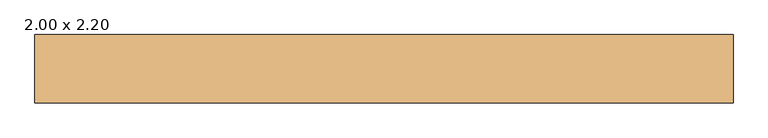
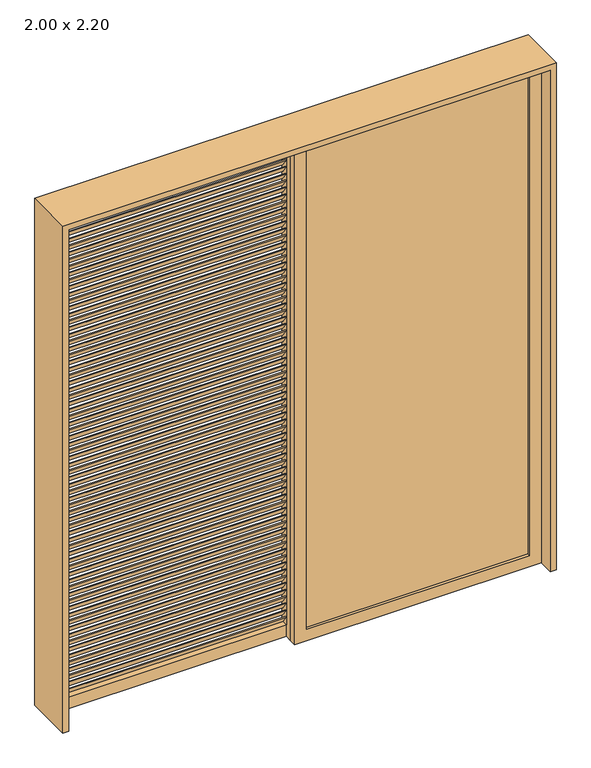
"""IFC4 building model written with IfcOpenShell, lengths in millimetres: door geometry, CC_PORTA CORRER_2 FOLHAS VENEZIANA + 1 FOLHA VIDRO : 2.00 x 2.20."""

from ifc_helpers import new_model, si_unit, frame, origin, place, context, project, spatial, polyline, outline, extrude, source, transform, mapped, element, save


def door_2_00_x_2_20_6a46caad(model_context):
    return source(origin(), model_context, "Body", "SweptSolid", [
        extrude(outline(polyline([(950.0, -26.0), (950.0, -34.0), (25.0, -34.0), (25.0, -26.0), (950.0, -26.0)])), frame((0.0, 0.0, 50.0), z_axis=(0.0, 0.0, 1.0), x_axis=(1.0, 0.0, 0.0)), (0.0, 0.0, 1.0), 2100.0),
        extrude(outline(polyline([(2200.0, 1000.0), (2200.0, -25.0), (0.0, -25.0), (0.0, 1000.0), (2200.0, 1000.0)]), holes=[polyline([(2150.0, 950.0), (50.0, 950.0), (50.0, 25.0), (2150.0, 25.0), (2150.0, 950.0)])]), frame((0.0, -45.0, 0.0), z_axis=(0.0, 1.0, 0.0), x_axis=(0.0, 0.0, 1.0)), (0.0, 0.0, 1.0), 30.0),
        extrude(outline(polyline([(40.0, 2085.0724638), (15.0, 2120.0724638), (20.0, 2120.0724638), (45.0, 2085.0724638), (40.0, 2085.0724638)])), frame((-950.0, 0.0, 0.0), z_axis=(1.0, 0.0, 0.0), x_axis=(0.0, 1.0, 0.0)), (0.0, 0.0, 1.0), 925.0),
        extrude(outline(polyline([(40.0, 2055.1449275), (15.0, 2090.1449275), (20.0, 2090.1449275), (45.0, 2055.1449275), (40.0, 2055.1449275)])), frame((-950.0, 0.0, 0.0), z_axis=(1.0, 0.0, 0.0), x_axis=(0.0, 1.0, 0.0)), (0.0, 0.0, 1.0), 925.0),
        extrude(outline(polyline([(40.0, 2025.2173913), (15.0, 2060.2173913), (20.0, 2060.2173913), (45.0, 2025.2173913), (40.0, 2025.2173913)])), frame((-950.0, 0.0, 0.0), z_axis=(1.0, 0.0, 0.0), x_axis=(0.0, 1.0, 0.0)), (0.0, 0.0, 1.0), 925.0),
        extrude(outline(polyline([(40.0, 1995.2898551), (15.0, 2030.2898551), (20.0, 2030.2898551), (45.0, 1995.2898551), (40.0, 1995.2898551)])), frame((-950.0, 0.0, 0.0), z_axis=(1.0, 0.0, 0.0), x_axis=(0.0, 1.0, 0.0)), (0.0, 0.0, 1.0), 925.0),
        extrude(outline(polyline([(40.0, 1965.3623188), (15.0, 2000.3623188), (20.0, 2000.3623188), (45.0, 1965.3623188), (40.0, 1965.3623188)])), frame((-950.0, 0.0, 0.0), z_axis=(1.0, 0.0, 0.0), x_axis=(0.0, 1.0, 0.0)), (0.0, 0.0, 1.0), 925.0),
        extrude(outline(polyline([(40.0, 1935.4347826), (15.0, 1970.4347826), (20.0, 1970.4347826), (45.0, 1935.4347826), (40.0, 1935.4347826)])), frame((-950.0, 0.0, 0.0), z_axis=(1.0, 0.0, 0.0), x_axis=(0.0, 1.0, 0.0)), (0.0, 0.0, 1.0), 925.0),
        extrude(outline(polyline([(40.0, 1905.5072464), (15.0, 1940.5072464), (20.0, 1940.5072464), (45.0, 1905.5072464), (40.0, 1905.5072464)])), frame((-950.0, 0.0, 0.0), z_axis=(1.0, 0.0, 0.0), x_axis=(0.0, 1.0, 0.0)), (0.0, 0.0, 1.0), 925.0),
        extrude(outline(polyline([(40.0, 1875.5797101), (15.0, 1910.5797101), (20.0, 1910.5797101), (45.0, 1875.5797101), (40.0, 1875.5797101)])), frame((-950.0, 0.0, 0.0), z_axis=(1.0, 0.0, 0.0), x_axis=(0.0, 1.0, 0.0)), (0.0, 0.0, 1.0), 925.0),
        extrude(outline(polyline([(40.0, 1845.6521739), (15.0, 1880.6521739), (20.0, 1880.6521739), (45.0, 1845.6521739), (40.0, 1845.6521739)])), frame((-950.0, 0.0, 0.0), z_axis=(1.0, 0.0, 0.0), x_axis=(0.0, 1.0, 0.0)), (0.0, 0.0, 1.0), 925.0),
        extrude(outline(polyline([(40.0, 1815.7246377), (15.0, 1850.7246377), (20.0, 1850.7246377), (45.0, 1815.7246377), (40.0, 1815.7246377)])), frame((-950.0, 0.0, 0.0), z_axis=(1.0, 0.0, 0.0), x_axis=(0.0, 1.0, 0.0)), (0.0, 0.0, 1.0), 925.0),
        extrude(outline(polyline([(40.0, 1785.7971014), (15.0, 1820.7971014), (20.0, 1820.7971014), (45.0, 1785.7971014), (40.0, 1785.7971014)])), frame((-950.0, 0.0, 0.0), z_axis=(1.0, 0.0, 0.0), x_axis=(0.0, 1.0, 0.0)), (0.0, 0.0, 1.0), 925.0),
        extrude(outline(polyline([(40.0, 1755.8695652), (15.0, 1790.8695652), (20.0, 1790.8695652), (45.0, 1755.8695652), (40.0, 1755.8695652)])), frame((-950.0, 0.0, 0.0), z_axis=(1.0, 0.0, 0.0), x_axis=(0.0, 1.0, 0.0)), (0.0, 0.0, 1.0), 925.0),
        extrude(outline(polyline([(40.0, 1725.942029), (15.0, 1760.942029), (20.0, 1760.942029), (45.0, 1725.942029), (40.0, 1725.942029)])), frame((-950.0, 0.0, 0.0), z_axis=(1.0, 0.0, 0.0), x_axis=(0.0, 1.0, 0.0)), (0.0, 0.0, 1.0), 925.0),
        extrude(outline(polyline([(40.0, 1696.0144928), (15.0, 1731.0144928), (20.0, 1731.0144928), (45.0, 1696.0144928), (40.0, 1696.0144928)])), frame((-950.0, 0.0, 0.0), z_axis=(1.0, 0.0, 0.0), x_axis=(0.0, 1.0, 0.0)), (0.0, 0.0, 1.0), 925.0),
        extrude(outline(polyline([(40.0, 1666.0869565), (15.0, 1701.0869565), (20.0, 1701.0869565), (45.0, 1666.0869565), (40.0, 1666.0869565)])), frame((-950.0, 0.0, 0.0), z_axis=(1.0, 0.0, 0.0), x_axis=(0.0, 1.0, 0.0)), (0.0, 0.0, 1.0), 925.0),
        extrude(outline(polyline([(40.0, 1636.1594203), (15.0, 1671.1594203), (20.0, 1671.1594203), (45.0, 1636.1594203), (40.0, 1636.1594203)])), frame((-950.0, 0.0, 0.0), z_axis=(1.0, 0.0, 0.0), x_axis=(0.0, 1.0, 0.0)), (0.0, 0.0, 1.0), 925.0),
        extrude(outline(polyline([(40.0, 1606.2318841), (15.0, 1641.2318841), (20.0, 1641.2318841), (45.0, 1606.2318841), (40.0, 1606.2318841)])), frame((-950.0, 0.0, 0.0), z_axis=(1.0, 0.0, 0.0), x_axis=(0.0, 1.0, 0.0)), (0.0, 0.0, 1.0), 925.0),
        extrude(outline(polyline([(40.0, 1576.3043478), (15.0, 1611.3043478), (20.0, 1611.3043478), (45.0, 1576.3043478), (40.0, 1576.3043478)])), frame((-950.0, 0.0, 0.0), z_axis=(1.0, 0.0, 0.0), x_axis=(0.0, 1.0, 0.0)), (0.0, 0.0, 1.0), 925.0),
        extrude(outline(polyline([(40.0, 1546.3768116), (15.0, 1581.3768116), (20.0, 1581.3768116), (45.0, 1546.3768116), (40.0, 1546.3768116)])), frame((-950.0, 0.0, 0.0), z_axis=(1.0, 0.0, 0.0), x_axis=(0.0, 1.0, 0.0)), (0.0, 0.0, 1.0), 925.0),
        extrude(outline(polyline([(40.0, 1516.4492754), (15.0, 1551.4492754), (20.0, 1551.4492754), (45.0, 1516.4492754), (40.0, 1516.4492754)])), frame((-950.0, 0.0, 0.0), z_axis=(1.0, 0.0, 0.0), x_axis=(0.0, 1.0, 0.0)), (0.0, 0.0, 1.0), 925.0),
        extrude(outline(polyline([(40.0, 1486.5217391), (15.0, 1521.5217391), (20.0, 1521.5217391), (45.0, 1486.5217391), (40.0, 1486.5217391)])), frame((-950.0, 0.0, 0.0), z_axis=(1.0, 0.0, 0.0), x_axis=(0.0, 1.0, 0.0)), (0.0, 0.0, 1.0), 925.0),
        extrude(outline(polyline([(40.0, 1456.5942029), (15.0, 1491.5942029), (20.0, 1491.5942029), (45.0, 1456.5942029), (40.0, 1456.5942029)])), frame((-950.0, 0.0, 0.0), z_axis=(1.0, 0.0, 0.0), x_axis=(0.0, 1.0, 0.0)), (0.0, 0.0, 1.0), 925.0),
        extrude(outline(polyline([(40.0, 1426.6666667), (15.0, 1461.6666667), (20.0, 1461.6666667), (45.0, 1426.6666667), (40.0, 1426.6666667)])), frame((-950.0, 0.0, 0.0), z_axis=(1.0, 0.0, 0.0), x_axis=(0.0, 1.0, 0.0)), (0.0, 0.0, 1.0), 925.0),
        extrude(outline(polyline([(40.0, 1396.7391304), (15.0, 1431.7391304), (20.0, 1431.7391304), (45.0, 1396.7391304), (40.0, 1396.7391304)])), frame((-950.0, 0.0, 0.0), z_axis=(1.0, 0.0, 0.0), x_axis=(0.0, 1.0, 0.0)), (0.0, 0.0, 1.0), 925.0),
        extrude(outline(polyline([(40.0, 1366.8115942), (15.0, 1401.8115942), (20.0, 1401.8115942), (45.0, 1366.8115942), (40.0, 1366.8115942)])), frame((-950.0, 0.0, 0.0), z_axis=(1.0, 0.0, 0.0), x_axis=(0.0, 1.0, 0.0)), (0.0, 0.0, 1.0), 925.0),
        extrude(outline(polyline([(40.0, 1336.884058), (15.0, 1371.884058), (20.0, 1371.884058), (45.0, 1336.884058), (40.0, 1336.884058)])), frame((-950.0, 0.0, 0.0), z_axis=(1.0, 0.0, 0.0), x_axis=(0.0, 1.0, 0.0)), (0.0, 0.0, 1.0), 925.0),
        extrude(outline(polyline([(40.0, 1306.9565217), (15.0, 1341.9565217), (20.0, 1341.9565217), (45.0, 1306.9565217), (40.0, 1306.9565217)])), frame((-950.0, 0.0, 0.0), z_axis=(1.0, 0.0, 0.0), x_axis=(0.0, 1.0, 0.0)), (0.0, 0.0, 1.0), 925.0),
        extrude(outline(polyline([(40.0, 1277.0289855), (15.0, 1312.0289855), (20.0, 1312.0289855), (45.0, 1277.0289855), (40.0, 1277.0289855)])), frame((-950.0, 0.0, 0.0), z_axis=(1.0, 0.0, 0.0), x_axis=(0.0, 1.0, 0.0)), (0.0, 0.0, 1.0), 925.0),
        extrude(outline(polyline([(40.0, 1247.1014493), (15.0, 1282.1014493), (20.0, 1282.1014493), (45.0, 1247.1014493), (40.0, 1247.1014493)])), frame((-950.0, 0.0, 0.0), z_axis=(1.0, 0.0, 0.0), x_axis=(0.0, 1.0, 0.0)), (0.0, 0.0, 1.0), 925.0),
        extrude(outline(polyline([(40.0, 1217.173913), (15.0, 1252.173913), (20.0, 1252.173913), (45.0, 1217.173913), (40.0, 1217.173913)])), frame((-950.0, 0.0, 0.0), z_axis=(1.0, 0.0, 0.0), x_axis=(0.0, 1.0, 0.0)), (0.0, 0.0, 1.0), 925.0),
        extrude(outline(polyline([(40.0, 1187.2463768), (15.0, 1222.2463768), (20.0, 1222.2463768), (45.0, 1187.2463768), (40.0, 1187.2463768)])), frame((-950.0, 0.0, 0.0), z_axis=(1.0, 0.0, 0.0), x_axis=(0.0, 1.0, 0.0)), (0.0, 0.0, 1.0), 925.0),
        extrude(outline(polyline([(40.0, 1157.3188406), (15.0, 1192.3188406), (20.0, 1192.3188406), (45.0, 1157.3188406), (40.0, 1157.3188406)])), frame((-950.0, 0.0, 0.0), z_axis=(1.0, 0.0, 0.0), x_axis=(0.0, 1.0, 0.0)), (0.0, 0.0, 1.0), 925.0),
        extrude(outline(polyline([(40.0, 1127.3913043), (15.0, 1162.3913043), (20.0, 1162.3913043), (45.0, 1127.3913043), (40.0, 1127.3913043)])), frame((-950.0, 0.0, 0.0), z_axis=(1.0, 0.0, 0.0), x_axis=(0.0, 1.0, 0.0)), (0.0, 0.0, 1.0), 925.0),
        extrude(outline(polyline([(40.0, 1097.4637681), (15.0, 1132.4637681), (20.0, 1132.4637681), (45.0, 1097.4637681), (40.0, 1097.4637681)])), frame((-950.0, 0.0, 0.0), z_axis=(1.0, 0.0, 0.0), x_axis=(0.0, 1.0, 0.0)), (0.0, 0.0, 1.0), 925.0),
        extrude(outline(polyline([(40.0, 1067.5362319), (15.0, 1102.5362319), (20.0, 1102.5362319), (45.0, 1067.5362319), (40.0, 1067.5362319)])), frame((-950.0, 0.0, 0.0), z_axis=(1.0, 0.0, 0.0), x_axis=(0.0, 1.0, 0.0)), (0.0, 0.0, 1.0), 925.0),
        extrude(outline(polyline([(40.0, 1037.6086957), (15.0, 1072.6086957), (20.0, 1072.6086957), (45.0, 1037.6086957), (40.0, 1037.6086957)])), frame((-950.0, 0.0, 0.0), z_axis=(1.0, 0.0, 0.0), x_axis=(0.0, 1.0, 0.0)), (0.0, 0.0, 1.0), 925.0),
        extrude(outline(polyline([(40.0, 1007.6811594), (15.0, 1042.6811594), (20.0, 1042.6811594), (45.0, 1007.6811594), (40.0, 1007.6811594)])), frame((-950.0, 0.0, 0.0), z_axis=(1.0, 0.0, 0.0), x_axis=(0.0, 1.0, 0.0)), (0.0, 0.0, 1.0), 925.0),
        extrude(outline(polyline([(40.0, 977.7536232), (15.0, 1012.7536232), (20.0, 1012.7536232), (45.0, 977.7536232), (40.0, 977.7536232)])), frame((-950.0, 0.0, 0.0), z_axis=(1.0, 0.0, 0.0), x_axis=(0.0, 1.0, 0.0)), (0.0, 0.0, 1.0), 925.0),
        extrude(outline(polyline([(40.0, 947.826087), (15.0, 982.826087), (20.0, 982.826087), (45.0, 947.826087), (40.0, 947.826087)])), frame((-950.0, 0.0, 0.0), z_axis=(1.0, 0.0, 0.0), x_axis=(0.0, 1.0, 0.0)), (0.0, 0.0, 1.0), 925.0),
        extrude(outline(polyline([(40.0, 917.8985507), (15.0, 952.8985507), (20.0, 952.8985507), (45.0, 917.8985507), (40.0, 917.8985507)])), frame((-950.0, 0.0, 0.0), z_axis=(1.0, 0.0, 0.0), x_axis=(0.0, 1.0, 0.0)), (0.0, 0.0, 1.0), 925.0),
        extrude(outline(polyline([(40.0, 887.9710145), (15.0, 922.9710145), (20.0, 922.9710145), (45.0, 887.9710145), (40.0, 887.9710145)])), frame((-950.0, 0.0, 0.0), z_axis=(1.0, 0.0, 0.0), x_axis=(0.0, 1.0, 0.0)), (0.0, 0.0, 1.0), 925.0),
        extrude(outline(polyline([(40.0, 858.0434783), (15.0, 893.0434783), (20.0, 893.0434783), (45.0, 858.0434783), (40.0, 858.0434783)])), frame((-950.0, 0.0, 0.0), z_axis=(1.0, 0.0, 0.0), x_axis=(0.0, 1.0, 0.0)), (0.0, 0.0, 1.0), 925.0),
        extrude(outline(polyline([(40.0, 828.115942), (15.0, 863.115942), (20.0, 863.115942), (45.0, 828.115942), (40.0, 828.115942)])), frame((-950.0, 0.0, 0.0), z_axis=(1.0, 0.0, 0.0), x_axis=(0.0, 1.0, 0.0)), (0.0, 0.0, 1.0), 925.0),
        extrude(outline(polyline([(40.0, 798.1884058), (15.0, 833.1884058), (20.0, 833.1884058), (45.0, 798.1884058), (40.0, 798.1884058)])), frame((-950.0, 0.0, 0.0), z_axis=(1.0, 0.0, 0.0), x_axis=(0.0, 1.0, 0.0)), (0.0, 0.0, 1.0), 925.0),
        extrude(outline(polyline([(40.0, 768.2608696), (15.0, 803.2608696), (20.0, 803.2608696), (45.0, 768.2608696), (40.0, 768.2608696)])), frame((-950.0, 0.0, 0.0), z_axis=(1.0, 0.0, 0.0), x_axis=(0.0, 1.0, 0.0)), (0.0, 0.0, 1.0), 925.0),
        extrude(outline(polyline([(40.0, 738.3333333), (15.0, 773.3333333), (20.0, 773.3333333), (45.0, 738.3333333), (40.0, 738.3333333)])), frame((-950.0, 0.0, 0.0), z_axis=(1.0, 0.0, 0.0), x_axis=(0.0, 1.0, 0.0)), (0.0, 0.0, 1.0), 925.0),
        extrude(outline(polyline([(40.0, 708.4057971), (15.0, 743.4057971), (20.0, 743.4057971), (45.0, 708.4057971), (40.0, 708.4057971)])), frame((-950.0, 0.0, 0.0), z_axis=(1.0, 0.0, 0.0), x_axis=(0.0, 1.0, 0.0)), (0.0, 0.0, 1.0), 925.0),
        extrude(outline(polyline([(40.0, 678.4782609), (15.0, 713.4782609), (20.0, 713.4782609), (45.0, 678.4782609), (40.0, 678.4782609)])), frame((-950.0, 0.0, 0.0), z_axis=(1.0, 0.0, 0.0), x_axis=(0.0, 1.0, 0.0)), (0.0, 0.0, 1.0), 925.0),
        extrude(outline(polyline([(40.0, 648.5507246), (15.0, 683.5507246), (20.0, 683.5507246), (45.0, 648.5507246), (40.0, 648.5507246)])), frame((-950.0, 0.0, 0.0), z_axis=(1.0, 0.0, 0.0), x_axis=(0.0, 1.0, 0.0)), (0.0, 0.0, 1.0), 925.0),
        extrude(outline(polyline([(40.0, 618.6231884), (15.0, 653.6231884), (20.0, 653.6231884), (45.0, 618.6231884), (40.0, 618.6231884)])), frame((-950.0, 0.0, 0.0), z_axis=(1.0, 0.0, 0.0), x_axis=(0.0, 1.0, 0.0)), (0.0, 0.0, 1.0), 925.0),
        extrude(outline(polyline([(40.0, 588.6956522), (15.0, 623.6956522), (20.0, 623.6956522), (45.0, 588.6956522), (40.0, 588.6956522)])), frame((-950.0, 0.0, 0.0), z_axis=(1.0, 0.0, 0.0), x_axis=(0.0, 1.0, 0.0)), (0.0, 0.0, 1.0), 925.0),
        extrude(outline(polyline([(40.0, 558.7681159), (15.0, 593.7681159), (20.0, 593.7681159), (45.0, 558.7681159), (40.0, 558.7681159)])), frame((-950.0, 0.0, 0.0), z_axis=(1.0, 0.0, 0.0), x_axis=(0.0, 1.0, 0.0)), (0.0, 0.0, 1.0), 925.0),
        extrude(outline(polyline([(40.0, 528.8405797), (15.0, 563.8405797), (20.0, 563.8405797), (45.0, 528.8405797), (40.0, 528.8405797)])), frame((-950.0, 0.0, 0.0), z_axis=(1.0, 0.0, 0.0), x_axis=(0.0, 1.0, 0.0)), (0.0, 0.0, 1.0), 925.0),
        extrude(outline(polyline([(40.0, 498.9130435), (15.0, 533.9130435), (20.0, 533.9130435), (45.0, 498.9130435), (40.0, 498.9130435)])), frame((-950.0, 0.0, 0.0), z_axis=(1.0, 0.0, 0.0), x_axis=(0.0, 1.0, 0.0)), (0.0, 0.0, 1.0), 925.0),
        extrude(outline(polyline([(40.0, 468.9855072), (15.0, 503.9855072), (20.0, 503.9855072), (45.0, 468.9855072), (40.0, 468.9855072)])), frame((-950.0, 0.0, 0.0), z_axis=(1.0, 0.0, 0.0), x_axis=(0.0, 1.0, 0.0)), (0.0, 0.0, 1.0), 925.0),
        extrude(outline(polyline([(40.0, 439.057971), (15.0, 474.057971), (20.0, 474.057971), (45.0, 439.057971), (40.0, 439.057971)])), frame((-950.0, 0.0, 0.0), z_axis=(1.0, 0.0, 0.0), x_axis=(0.0, 1.0, 0.0)), (0.0, 0.0, 1.0), 925.0),
        extrude(outline(polyline([(40.0, 409.1304348), (15.0, 444.1304348), (20.0, 444.1304348), (45.0, 409.1304348), (40.0, 409.1304348)])), frame((-950.0, 0.0, 0.0), z_axis=(1.0, 0.0, 0.0), x_axis=(0.0, 1.0, 0.0)), (0.0, 0.0, 1.0), 925.0),
        extrude(outline(polyline([(40.0, 379.2028986), (15.0, 414.2028986), (20.0, 414.2028986), (45.0, 379.2028986), (40.0, 379.2028986)])), frame((-950.0, 0.0, 0.0), z_axis=(1.0, 0.0, 0.0), x_axis=(0.0, 1.0, 0.0)), (0.0, 0.0, 1.0), 925.0),
        extrude(outline(polyline([(40.0, 349.2753623), (15.0, 384.2753623), (20.0, 384.2753623), (45.0, 349.2753623), (40.0, 349.2753623)])), frame((-950.0, 0.0, 0.0), z_axis=(1.0, 0.0, 0.0), x_axis=(0.0, 1.0, 0.0)), (0.0, 0.0, 1.0), 925.0),
        extrude(outline(polyline([(40.0, 319.3478261), (15.0, 354.3478261), (20.0, 354.3478261), (45.0, 319.3478261), (40.0, 319.3478261)])), frame((-950.0, 0.0, 0.0), z_axis=(1.0, 0.0, 0.0), x_axis=(0.0, 1.0, 0.0)), (0.0, 0.0, 1.0), 925.0),
        extrude(outline(polyline([(40.0, 289.4202899), (15.0, 324.4202899), (20.0, 324.4202899), (45.0, 289.4202899), (40.0, 289.4202899)])), frame((-950.0, 0.0, 0.0), z_axis=(1.0, 0.0, 0.0), x_axis=(0.0, 1.0, 0.0)), (0.0, 0.0, 1.0), 925.0),
        extrude(outline(polyline([(40.0, 259.4927536), (15.0, 294.4927536), (20.0, 294.4927536), (45.0, 259.4927536), (40.0, 259.4927536)])), frame((-950.0, 0.0, 0.0), z_axis=(1.0, 0.0, 0.0), x_axis=(0.0, 1.0, 0.0)), (0.0, 0.0, 1.0), 925.0),
        extrude(outline(polyline([(40.0, 229.5652174), (15.0, 264.5652174), (20.0, 264.5652174), (45.0, 229.5652174), (40.0, 229.5652174)])), frame((-950.0, 0.0, 0.0), z_axis=(1.0, 0.0, 0.0), x_axis=(0.0, 1.0, 0.0)), (0.0, 0.0, 1.0), 925.0),
        extrude(outline(polyline([(40.0, 199.6376812), (15.0, 234.6376812), (20.0, 234.6376812), (45.0, 199.6376812), (40.0, 199.6376812)])), frame((-950.0, 0.0, 0.0), z_axis=(1.0, 0.0, 0.0), x_axis=(0.0, 1.0, 0.0)), (0.0, 0.0, 1.0), 925.0),
        extrude(outline(polyline([(40.0, 169.7101449), (15.0, 204.7101449), (20.0, 204.7101449), (45.0, 169.7101449), (40.0, 169.7101449)])), frame((-950.0, 0.0, 0.0), z_axis=(1.0, 0.0, 0.0), x_axis=(0.0, 1.0, 0.0)), (0.0, 0.0, 1.0), 925.0),
        extrude(outline(polyline([(40.0, 139.7826087), (15.0, 174.7826087), (20.0, 174.7826087), (45.0, 139.7826087), (40.0, 139.7826087)])), frame((-950.0, 0.0, 0.0), z_axis=(1.0, 0.0, 0.0), x_axis=(0.0, 1.0, 0.0)), (0.0, 0.0, 1.0), 925.0),
        extrude(outline(polyline([(40.0, 109.8550725), (15.0, 144.8550725), (20.0, 144.8550725), (45.0, 109.8550725), (40.0, 109.8550725)])), frame((-950.0, 0.0, 0.0), z_axis=(1.0, 0.0, 0.0), x_axis=(0.0, 1.0, 0.0)), (0.0, 0.0, 1.0), 925.0),
        extrude(outline(polyline([(40.0, 79.9275362), (15.0, 114.9275362), (20.0, 114.9275362), (45.0, 79.9275362), (40.0, 79.9275362)])), frame((-950.0, 0.0, 0.0), z_axis=(1.0, 0.0, 0.0), x_axis=(0.0, 1.0, 0.0)), (0.0, 0.0, 1.0), 925.0),
        extrude(outline(polyline([(40.0, 2115.0), (15.0, 2150.0), (20.0, 2150.0), (45.0, 2115.0), (40.0, 2115.0)])), frame((-950.0, 0.0, 0.0), z_axis=(1.0, 0.0, 0.0), x_axis=(0.0, 1.0, 0.0)), (0.0, 0.0, 1.0), 925.0),
        extrude(outline(polyline([(40.0, 50.0), (15.0, 85.0), (20.0, 85.0), (45.0, 50.0), (40.0, 50.0)])), frame((-950.0, 0.0, 0.0), z_axis=(1.0, 0.0, 0.0), x_axis=(0.0, 1.0, 0.0)), (0.0, 0.0, 1.0), 925.0),
        extrude(outline(polyline([(2200.0, 25.0), (2200.0, -1000.0), (0.0, -1000.0), (0.0, 25.0), (2200.0, 25.0)]), holes=[polyline([(2150.0, -25.0), (50.0, -25.0), (50.0, -950.0), (2150.0, -950.0), (2150.0, -25.0)])]), frame((0.0, 15.0, 0.0), z_axis=(0.0, 1.0, 0.0), x_axis=(0.0, 0.0, 1.0)), (0.0, 0.0, 1.0), 30.0),
        extrude(outline(polyline([(10.0, 2085.0724638), (-15.0, 2120.0724638), (-10.0, 2120.0724638), (15.0, 2085.0724638), (10.0, 2085.0724638)])), frame((25.0, 0.0, 0.0), z_axis=(1.0, 0.0, 0.0), x_axis=(0.0, 1.0, 0.0)), (0.0, 0.0, 1.0), 925.0),
        extrude(outline(polyline([(10.0, 2055.1449275), (-15.0, 2090.1449275), (-10.0, 2090.1449275), (15.0, 2055.1449275), (10.0, 2055.1449275)])), frame((25.0, 0.0, 0.0), z_axis=(1.0, 0.0, 0.0), x_axis=(0.0, 1.0, 0.0)), (0.0, 0.0, 1.0), 925.0),
        extrude(outline(polyline([(10.0, 2025.2173913), (-15.0, 2060.2173913), (-10.0, 2060.2173913), (15.0, 2025.2173913), (10.0, 2025.2173913)])), frame((25.0, 0.0, 0.0), z_axis=(1.0, 0.0, 0.0), x_axis=(0.0, 1.0, 0.0)), (0.0, 0.0, 1.0), 925.0),
        extrude(outline(polyline([(10.0, 1995.2898551), (-15.0, 2030.2898551), (-10.0, 2030.2898551), (15.0, 1995.2898551), (10.0, 1995.2898551)])), frame((25.0, 0.0, 0.0), z_axis=(1.0, 0.0, 0.0), x_axis=(0.0, 1.0, 0.0)), (0.0, 0.0, 1.0), 925.0),
        extrude(outline(polyline([(10.0, 1965.3623188), (-15.0, 2000.3623188), (-10.0, 2000.3623188), (15.0, 1965.3623188), (10.0, 1965.3623188)])), frame((25.0, 0.0, 0.0), z_axis=(1.0, 0.0, 0.0), x_axis=(0.0, 1.0, 0.0)), (0.0, 0.0, 1.0), 925.0),
        extrude(outline(polyline([(10.0, 1935.4347826), (-15.0, 1970.4347826), (-10.0, 1970.4347826), (15.0, 1935.4347826), (10.0, 1935.4347826)])), frame((25.0, 0.0, 0.0), z_axis=(1.0, 0.0, 0.0), x_axis=(0.0, 1.0, 0.0)), (0.0, 0.0, 1.0), 925.0),
        extrude(outline(polyline([(10.0, 1905.5072464), (-15.0, 1940.5072464), (-10.0, 1940.5072464), (15.0, 1905.5072464), (10.0, 1905.5072464)])), frame((25.0, 0.0, 0.0), z_axis=(1.0, 0.0, 0.0), x_axis=(0.0, 1.0, 0.0)), (0.0, 0.0, 1.0), 925.0),
        extrude(outline(polyline([(10.0, 1875.5797101), (-15.0, 1910.5797101), (-10.0, 1910.5797101), (15.0, 1875.5797101), (10.0, 1875.5797101)])), frame((25.0, 0.0, 0.0), z_axis=(1.0, 0.0, 0.0), x_axis=(0.0, 1.0, 0.0)), (0.0, 0.0, 1.0), 925.0),
        extrude(outline(polyline([(10.0, 1845.6521739), (-15.0, 1880.6521739), (-10.0, 1880.6521739), (15.0, 1845.6521739), (10.0, 1845.6521739)])), frame((25.0, 0.0, 0.0), z_axis=(1.0, 0.0, 0.0), x_axis=(0.0, 1.0, 0.0)), (0.0, 0.0, 1.0), 925.0),
        extrude(outline(polyline([(10.0, 1815.7246377), (-15.0, 1850.7246377), (-10.0, 1850.7246377), (15.0, 1815.7246377), (10.0, 1815.7246377)])), frame((25.0, 0.0, 0.0), z_axis=(1.0, 0.0, 0.0), x_axis=(0.0, 1.0, 0.0)), (0.0, 0.0, 1.0), 925.0),
        extrude(outline(polyline([(10.0, 1785.7971014), (-15.0, 1820.7971014), (-10.0, 1820.7971014), (15.0, 1785.7971014), (10.0, 1785.7971014)])), frame((25.0, 0.0, 0.0), z_axis=(1.0, 0.0, 0.0), x_axis=(0.0, 1.0, 0.0)), (0.0, 0.0, 1.0), 925.0),
        extrude(outline(polyline([(10.0, 1755.8695652), (-15.0, 1790.8695652), (-10.0, 1790.8695652), (15.0, 1755.8695652), (10.0, 1755.8695652)])), frame((25.0, 0.0, 0.0), z_axis=(1.0, 0.0, 0.0), x_axis=(0.0, 1.0, 0.0)), (0.0, 0.0, 1.0), 925.0),
        extrude(outline(polyline([(10.0, 1725.942029), (-15.0, 1760.942029), (-10.0, 1760.942029), (15.0, 1725.942029), (10.0, 1725.942029)])), frame((25.0, 0.0, 0.0), z_axis=(1.0, 0.0, 0.0), x_axis=(0.0, 1.0, 0.0)), (0.0, 0.0, 1.0), 925.0),
        extrude(outline(polyline([(10.0, 1696.0144928), (-15.0, 1731.0144928), (-10.0, 1731.0144928), (15.0, 1696.0144928), (10.0, 1696.0144928)])), frame((25.0, 0.0, 0.0), z_axis=(1.0, 0.0, 0.0), x_axis=(0.0, 1.0, 0.0)), (0.0, 0.0, 1.0), 925.0),
        extrude(outline(polyline([(10.0, 1666.0869565), (-15.0, 1701.0869565), (-10.0, 1701.0869565), (15.0, 1666.0869565), (10.0, 1666.0869565)])), frame((25.0, 0.0, 0.0), z_axis=(1.0, 0.0, 0.0), x_axis=(0.0, 1.0, 0.0)), (0.0, 0.0, 1.0), 925.0),
        extrude(outline(polyline([(10.0, 1636.1594203), (-15.0, 1671.1594203), (-10.0, 1671.1594203), (15.0, 1636.1594203), (10.0, 1636.1594203)])), frame((25.0, 0.0, 0.0), z_axis=(1.0, 0.0, 0.0), x_axis=(0.0, 1.0, 0.0)), (0.0, 0.0, 1.0), 925.0),
        extrude(outline(polyline([(10.0, 1606.2318841), (-15.0, 1641.2318841), (-10.0, 1641.2318841), (15.0, 1606.2318841), (10.0, 1606.2318841)])), frame((25.0, 0.0, 0.0), z_axis=(1.0, 0.0, 0.0), x_axis=(0.0, 1.0, 0.0)), (0.0, 0.0, 1.0), 925.0),
        extrude(outline(polyline([(10.0, 1576.3043478), (-15.0, 1611.3043478), (-10.0, 1611.3043478), (15.0, 1576.3043478), (10.0, 1576.3043478)])), frame((25.0, 0.0, 0.0), z_axis=(1.0, 0.0, 0.0), x_axis=(0.0, 1.0, 0.0)), (0.0, 0.0, 1.0), 925.0),
        extrude(outline(polyline([(10.0, 1546.3768116), (-15.0, 1581.3768116), (-10.0, 1581.3768116), (15.0, 1546.3768116), (10.0, 1546.3768116)])), frame((25.0, 0.0, 0.0), z_axis=(1.0, 0.0, 0.0), x_axis=(0.0, 1.0, 0.0)), (0.0, 0.0, 1.0), 925.0),
        extrude(outline(polyline([(10.0, 1516.4492754), (-15.0, 1551.4492754), (-10.0, 1551.4492754), (15.0, 1516.4492754), (10.0, 1516.4492754)])), frame((25.0, 0.0, 0.0), z_axis=(1.0, 0.0, 0.0), x_axis=(0.0, 1.0, 0.0)), (0.0, 0.0, 1.0), 925.0),
        extrude(outline(polyline([(10.0, 1486.5217391), (-15.0, 1521.5217391), (-10.0, 1521.5217391), (15.0, 1486.5217391), (10.0, 1486.5217391)])), frame((25.0, 0.0, 0.0), z_axis=(1.0, 0.0, 0.0), x_axis=(0.0, 1.0, 0.0)), (0.0, 0.0, 1.0), 925.0),
        extrude(outline(polyline([(10.0, 1456.5942029), (-15.0, 1491.5942029), (-10.0, 1491.5942029), (15.0, 1456.5942029), (10.0, 1456.5942029)])), frame((25.0, 0.0, 0.0), z_axis=(1.0, 0.0, 0.0), x_axis=(0.0, 1.0, 0.0)), (0.0, 0.0, 1.0), 925.0),
        extrude(outline(polyline([(10.0, 1426.6666667), (-15.0, 1461.6666667), (-10.0, 1461.6666667), (15.0, 1426.6666667), (10.0, 1426.6666667)])), frame((25.0, 0.0, 0.0), z_axis=(1.0, 0.0, 0.0), x_axis=(0.0, 1.0, 0.0)), (0.0, 0.0, 1.0), 925.0),
        extrude(outline(polyline([(10.0, 1396.7391304), (-15.0, 1431.7391304), (-10.0, 1431.7391304), (15.0, 1396.7391304), (10.0, 1396.7391304)])), frame((25.0, 0.0, 0.0), z_axis=(1.0, 0.0, 0.0), x_axis=(0.0, 1.0, 0.0)), (0.0, 0.0, 1.0), 925.0),
        extrude(outline(polyline([(10.0, 1366.8115942), (-15.0, 1401.8115942), (-10.0, 1401.8115942), (15.0, 1366.8115942), (10.0, 1366.8115942)])), frame((25.0, 0.0, 0.0), z_axis=(1.0, 0.0, 0.0), x_axis=(0.0, 1.0, 0.0)), (0.0, 0.0, 1.0), 925.0),
        extrude(outline(polyline([(10.0, 1336.884058), (-15.0, 1371.884058), (-10.0, 1371.884058), (15.0, 1336.884058), (10.0, 1336.884058)])), frame((25.0, 0.0, 0.0), z_axis=(1.0, 0.0, 0.0), x_axis=(0.0, 1.0, 0.0)), (0.0, 0.0, 1.0), 925.0),
        extrude(outline(polyline([(10.0, 1306.9565217), (-15.0, 1341.9565217), (-10.0, 1341.9565217), (15.0, 1306.9565217), (10.0, 1306.9565217)])), frame((25.0, 0.0, 0.0), z_axis=(1.0, 0.0, 0.0), x_axis=(0.0, 1.0, 0.0)), (0.0, 0.0, 1.0), 925.0),
        extrude(outline(polyline([(10.0, 1277.0289855), (-15.0, 1312.0289855), (-10.0, 1312.0289855), (15.0, 1277.0289855), (10.0, 1277.0289855)])), frame((25.0, 0.0, 0.0), z_axis=(1.0, 0.0, 0.0), x_axis=(0.0, 1.0, 0.0)), (0.0, 0.0, 1.0), 925.0),
        extrude(outline(polyline([(10.0, 1247.1014493), (-15.0, 1282.1014493), (-10.0, 1282.1014493), (15.0, 1247.1014493), (10.0, 1247.1014493)])), frame((25.0, 0.0, 0.0), z_axis=(1.0, 0.0, 0.0), x_axis=(0.0, 1.0, 0.0)), (0.0, 0.0, 1.0), 925.0),
        extrude(outline(polyline([(10.0, 1217.173913), (-15.0, 1252.173913), (-10.0, 1252.173913), (15.0, 1217.173913), (10.0, 1217.173913)])), frame((25.0, 0.0, 0.0), z_axis=(1.0, 0.0, 0.0), x_axis=(0.0, 1.0, 0.0)), (0.0, 0.0, 1.0), 925.0),
        extrude(outline(polyline([(10.0, 1187.2463768), (-15.0, 1222.2463768), (-10.0, 1222.2463768), (15.0, 1187.2463768), (10.0, 1187.2463768)])), frame((25.0, 0.0, 0.0), z_axis=(1.0, 0.0, 0.0), x_axis=(0.0, 1.0, 0.0)), (0.0, 0.0, 1.0), 925.0),
        extrude(outline(polyline([(10.0, 1157.3188406), (-15.0, 1192.3188406), (-10.0, 1192.3188406), (15.0, 1157.3188406), (10.0, 1157.3188406)])), frame((25.0, 0.0, 0.0), z_axis=(1.0, 0.0, 0.0), x_axis=(0.0, 1.0, 0.0)), (0.0, 0.0, 1.0), 925.0),
        extrude(outline(polyline([(10.0, 1127.3913043), (-15.0, 1162.3913043), (-10.0, 1162.3913043), (15.0, 1127.3913043), (10.0, 1127.3913043)])), frame((25.0, 0.0, 0.0), z_axis=(1.0, 0.0, 0.0), x_axis=(0.0, 1.0, 0.0)), (0.0, 0.0, 1.0), 925.0),
        extrude(outline(polyline([(10.0, 1097.4637681), (-15.0, 1132.4637681), (-10.0, 1132.4637681), (15.0, 1097.4637681), (10.0, 1097.4637681)])), frame((25.0, 0.0, 0.0), z_axis=(1.0, 0.0, 0.0), x_axis=(0.0, 1.0, 0.0)), (0.0, 0.0, 1.0), 925.0),
        extrude(outline(polyline([(10.0, 1067.5362319), (-15.0, 1102.5362319), (-10.0, 1102.5362319), (15.0, 1067.5362319), (10.0, 1067.5362319)])), frame((25.0, 0.0, 0.0), z_axis=(1.0, 0.0, 0.0), x_axis=(0.0, 1.0, 0.0)), (0.0, 0.0, 1.0), 925.0),
        extrude(outline(polyline([(10.0, 1037.6086957), (-15.0, 1072.6086957), (-10.0, 1072.6086957), (15.0, 1037.6086957), (10.0, 1037.6086957)])), frame((25.0, 0.0, 0.0), z_axis=(1.0, 0.0, 0.0), x_axis=(0.0, 1.0, 0.0)), (0.0, 0.0, 1.0), 925.0),
        extrude(outline(polyline([(10.0, 1007.6811594), (-15.0, 1042.6811594), (-10.0, 1042.6811594), (15.0, 1007.6811594), (10.0, 1007.6811594)])), frame((25.0, 0.0, 0.0), z_axis=(1.0, 0.0, 0.0), x_axis=(0.0, 1.0, 0.0)), (0.0, 0.0, 1.0), 925.0),
        extrude(outline(polyline([(10.0, 977.7536232), (-15.0, 1012.7536232), (-10.0, 1012.7536232), (15.0, 977.7536232), (10.0, 977.7536232)])), frame((25.0, 0.0, 0.0), z_axis=(1.0, 0.0, 0.0), x_axis=(0.0, 1.0, 0.0)), (0.0, 0.0, 1.0), 925.0),
        extrude(outline(polyline([(10.0, 947.826087), (-15.0, 982.826087), (-10.0, 982.826087), (15.0, 947.826087), (10.0, 947.826087)])), frame((25.0, 0.0, 0.0), z_axis=(1.0, 0.0, 0.0), x_axis=(0.0, 1.0, 0.0)), (0.0, 0.0, 1.0), 925.0),
        extrude(outline(polyline([(10.0, 917.8985507), (-15.0, 952.8985507), (-10.0, 952.8985507), (15.0, 917.8985507), (10.0, 917.8985507)])), frame((25.0, 0.0, 0.0), z_axis=(1.0, 0.0, 0.0), x_axis=(0.0, 1.0, 0.0)), (0.0, 0.0, 1.0), 925.0),
        extrude(outline(polyline([(10.0, 887.9710145), (-15.0, 922.9710145), (-10.0, 922.9710145), (15.0, 887.9710145), (10.0, 887.9710145)])), frame((25.0, 0.0, 0.0), z_axis=(1.0, 0.0, 0.0), x_axis=(0.0, 1.0, 0.0)), (0.0, 0.0, 1.0), 925.0),
        extrude(outline(polyline([(10.0, 858.0434783), (-15.0, 893.0434783), (-10.0, 893.0434783), (15.0, 858.0434783), (10.0, 858.0434783)])), frame((25.0, 0.0, 0.0), z_axis=(1.0, 0.0, 0.0), x_axis=(0.0, 1.0, 0.0)), (0.0, 0.0, 1.0), 925.0),
        extrude(outline(polyline([(10.0, 828.115942), (-15.0, 863.115942), (-10.0, 863.115942), (15.0, 828.115942), (10.0, 828.115942)])), frame((25.0, 0.0, 0.0), z_axis=(1.0, 0.0, 0.0), x_axis=(0.0, 1.0, 0.0)), (0.0, 0.0, 1.0), 925.0),
        extrude(outline(polyline([(10.0, 798.1884058), (-15.0, 833.1884058), (-10.0, 833.1884058), (15.0, 798.1884058), (10.0, 798.1884058)])), frame((25.0, 0.0, 0.0), z_axis=(1.0, 0.0, 0.0), x_axis=(0.0, 1.0, 0.0)), (0.0, 0.0, 1.0), 925.0),
        extrude(outline(polyline([(10.0, 768.2608696), (-15.0, 803.2608696), (-10.0, 803.2608696), (15.0, 768.2608696), (10.0, 768.2608696)])), frame((25.0, 0.0, 0.0), z_axis=(1.0, 0.0, 0.0), x_axis=(0.0, 1.0, 0.0)), (0.0, 0.0, 1.0), 925.0),
        extrude(outline(polyline([(10.0, 738.3333333), (-15.0, 773.3333333), (-10.0, 773.3333333), (15.0, 738.3333333), (10.0, 738.3333333)])), frame((25.0, 0.0, 0.0), z_axis=(1.0, 0.0, 0.0), x_axis=(0.0, 1.0, 0.0)), (0.0, 0.0, 1.0), 925.0),
        extrude(outline(polyline([(10.0, 708.4057971), (-15.0, 743.4057971), (-10.0, 743.4057971), (15.0, 708.4057971), (10.0, 708.4057971)])), frame((25.0, 0.0, 0.0), z_axis=(1.0, 0.0, 0.0), x_axis=(0.0, 1.0, 0.0)), (0.0, 0.0, 1.0), 925.0),
        extrude(outline(polyline([(10.0, 678.4782609), (-15.0, 713.4782609), (-10.0, 713.4782609), (15.0, 678.4782609), (10.0, 678.4782609)])), frame((25.0, 0.0, 0.0), z_axis=(1.0, 0.0, 0.0), x_axis=(0.0, 1.0, 0.0)), (0.0, 0.0, 1.0), 925.0),
        extrude(outline(polyline([(10.0, 648.5507246), (-15.0, 683.5507246), (-10.0, 683.5507246), (15.0, 648.5507246), (10.0, 648.5507246)])), frame((25.0, 0.0, 0.0), z_axis=(1.0, 0.0, 0.0), x_axis=(0.0, 1.0, 0.0)), (0.0, 0.0, 1.0), 925.0),
        extrude(outline(polyline([(10.0, 618.6231884), (-15.0, 653.6231884), (-10.0, 653.6231884), (15.0, 618.6231884), (10.0, 618.6231884)])), frame((25.0, 0.0, 0.0), z_axis=(1.0, 0.0, 0.0), x_axis=(0.0, 1.0, 0.0)), (0.0, 0.0, 1.0), 925.0),
        extrude(outline(polyline([(10.0, 588.6956522), (-15.0, 623.6956522), (-10.0, 623.6956522), (15.0, 588.6956522), (10.0, 588.6956522)])), frame((25.0, 0.0, 0.0), z_axis=(1.0, 0.0, 0.0), x_axis=(0.0, 1.0, 0.0)), (0.0, 0.0, 1.0), 925.0),
        extrude(outline(polyline([(10.0, 558.7681159), (-15.0, 593.7681159), (-10.0, 593.7681159), (15.0, 558.7681159), (10.0, 558.7681159)])), frame((25.0, 0.0, 0.0), z_axis=(1.0, 0.0, 0.0), x_axis=(0.0, 1.0, 0.0)), (0.0, 0.0, 1.0), 925.0),
        extrude(outline(polyline([(10.0, 528.8405797), (-15.0, 563.8405797), (-10.0, 563.8405797), (15.0, 528.8405797), (10.0, 528.8405797)])), frame((25.0, 0.0, 0.0), z_axis=(1.0, 0.0, 0.0), x_axis=(0.0, 1.0, 0.0)), (0.0, 0.0, 1.0), 925.0),
        extrude(outline(polyline([(10.0, 498.9130435), (-15.0, 533.9130435), (-10.0, 533.9130435), (15.0, 498.9130435), (10.0, 498.9130435)])), frame((25.0, 0.0, 0.0), z_axis=(1.0, 0.0, 0.0), x_axis=(0.0, 1.0, 0.0)), (0.0, 0.0, 1.0), 925.0),
        extrude(outline(polyline([(10.0, 468.9855072), (-15.0, 503.9855072), (-10.0, 503.9855072), (15.0, 468.9855072), (10.0, 468.9855072)])), frame((25.0, 0.0, 0.0), z_axis=(1.0, 0.0, 0.0), x_axis=(0.0, 1.0, 0.0)), (0.0, 0.0, 1.0), 925.0),
        extrude(outline(polyline([(10.0, 439.057971), (-15.0, 474.057971), (-10.0, 474.057971), (15.0, 439.057971), (10.0, 439.057971)])), frame((25.0, 0.0, 0.0), z_axis=(1.0, 0.0, 0.0), x_axis=(0.0, 1.0, 0.0)), (0.0, 0.0, 1.0), 925.0),
        extrude(outline(polyline([(10.0, 409.1304348), (-15.0, 444.1304348), (-10.0, 444.1304348), (15.0, 409.1304348), (10.0, 409.1304348)])), frame((25.0, 0.0, 0.0), z_axis=(1.0, 0.0, 0.0), x_axis=(0.0, 1.0, 0.0)), (0.0, 0.0, 1.0), 925.0),
        extrude(outline(polyline([(10.0, 379.2028986), (-15.0, 414.2028986), (-10.0, 414.2028986), (15.0, 379.2028986), (10.0, 379.2028986)])), frame((25.0, 0.0, 0.0), z_axis=(1.0, 0.0, 0.0), x_axis=(0.0, 1.0, 0.0)), (0.0, 0.0, 1.0), 925.0),
        extrude(outline(polyline([(10.0, 349.2753623), (-15.0, 384.2753623), (-10.0, 384.2753623), (15.0, 349.2753623), (10.0, 349.2753623)])), frame((25.0, 0.0, 0.0), z_axis=(1.0, 0.0, 0.0), x_axis=(0.0, 1.0, 0.0)), (0.0, 0.0, 1.0), 925.0),
        extrude(outline(polyline([(10.0, 319.3478261), (-15.0, 354.3478261), (-10.0, 354.3478261), (15.0, 319.3478261), (10.0, 319.3478261)])), frame((25.0, 0.0, 0.0), z_axis=(1.0, 0.0, 0.0), x_axis=(0.0, 1.0, 0.0)), (0.0, 0.0, 1.0), 925.0),
        extrude(outline(polyline([(10.0, 289.4202899), (-15.0, 324.4202899), (-10.0, 324.4202899), (15.0, 289.4202899), (10.0, 289.4202899)])), frame((25.0, 0.0, 0.0), z_axis=(1.0, 0.0, 0.0), x_axis=(0.0, 1.0, 0.0)), (0.0, 0.0, 1.0), 925.0),
        extrude(outline(polyline([(10.0, 259.4927536), (-15.0, 294.4927536), (-10.0, 294.4927536), (15.0, 259.4927536), (10.0, 259.4927536)])), frame((25.0, 0.0, 0.0), z_axis=(1.0, 0.0, 0.0), x_axis=(0.0, 1.0, 0.0)), (0.0, 0.0, 1.0), 925.0),
        extrude(outline(polyline([(10.0, 229.5652174), (-15.0, 264.5652174), (-10.0, 264.5652174), (15.0, 229.5652174), (10.0, 229.5652174)])), frame((25.0, 0.0, 0.0), z_axis=(1.0, 0.0, 0.0), x_axis=(0.0, 1.0, 0.0)), (0.0, 0.0, 1.0), 925.0),
        extrude(outline(polyline([(10.0, 199.6376812), (-15.0, 234.6376812), (-10.0, 234.6376812), (15.0, 199.6376812), (10.0, 199.6376812)])), frame((25.0, 0.0, 0.0), z_axis=(1.0, 0.0, 0.0), x_axis=(0.0, 1.0, 0.0)), (0.0, 0.0, 1.0), 925.0),
        extrude(outline(polyline([(10.0, 169.7101449), (-15.0, 204.7101449), (-10.0, 204.7101449), (15.0, 169.7101449), (10.0, 169.7101449)])), frame((25.0, 0.0, 0.0), z_axis=(1.0, 0.0, 0.0), x_axis=(0.0, 1.0, 0.0)), (0.0, 0.0, 1.0), 925.0),
        extrude(outline(polyline([(10.0, 139.7826087), (-15.0, 174.7826087), (-10.0, 174.7826087), (15.0, 139.7826087), (10.0, 139.7826087)])), frame((25.0, 0.0, 0.0), z_axis=(1.0, 0.0, 0.0), x_axis=(0.0, 1.0, 0.0)), (0.0, 0.0, 1.0), 925.0),
        extrude(outline(polyline([(10.0, 109.8550725), (-15.0, 144.8550725), (-10.0, 144.8550725), (15.0, 109.8550725), (10.0, 109.8550725)])), frame((25.0, 0.0, 0.0), z_axis=(1.0, 0.0, 0.0), x_axis=(0.0, 1.0, 0.0)), (0.0, 0.0, 1.0), 925.0),
        extrude(outline(polyline([(10.0, 79.9275362), (-15.0, 114.9275362), (-10.0, 114.9275362), (15.0, 79.9275362), (10.0, 79.9275362)])), frame((25.0, 0.0, 0.0), z_axis=(1.0, 0.0, 0.0), x_axis=(0.0, 1.0, 0.0)), (0.0, 0.0, 1.0), 925.0),
        extrude(outline(polyline([(10.0, 2115.0), (-15.0, 2150.0), (-10.0, 2150.0), (15.0, 2115.0), (10.0, 2115.0)])), frame((25.0, 0.0, 0.0), z_axis=(1.0, 0.0, 0.0), x_axis=(0.0, 1.0, 0.0)), (0.0, 0.0, 1.0), 925.0),
        extrude(outline(polyline([(10.0, 50.0), (-15.0, 85.0), (-10.0, 85.0), (15.0, 50.0), (10.0, 50.0)])), frame((25.0, 0.0, 0.0), z_axis=(1.0, 0.0, 0.0), x_axis=(0.0, 1.0, 0.0)), (0.0, 0.0, 1.0), 925.0),
        extrude(outline(polyline([(2200.0, 1000.0), (2200.0, -25.0), (0.0, -25.0), (0.0, 1000.0), (2200.0, 1000.0)]), holes=[polyline([(2150.0, 950.0), (50.0, 950.0), (50.0, 25.0), (2150.0, 25.0), (2150.0, 950.0)])]), frame((0.0, -15.0, 0.0), z_axis=(0.0, 1.0, 0.0), x_axis=(0.0, 0.0, 1.0)), (0.0, 0.0, 1.0), 30.0),
        extrude(outline(polyline([(0.0, -1025.0), (0.0, -1000.0), (2200.0, -1000.0), (2200.0, 1000.0), (0.0, 1000.0), (0.0, 1025.0), (2225.0, 1025.0), (2225.0, -1025.0), (0.0, -1025.0)])), frame((0.0, -107.5, 0.0), z_axis=(0.0, 1.0, 0.0), x_axis=(0.0, 0.0, 1.0)), (0.0, 0.0, 1.0), 200.0),
    ])


if __name__ == "__main__":
    model = new_model("IFC4")
    model_context = context("Model", 3, world=origin())
    ifc_project = project(units=[si_unit("LENGTHUNIT", "METRE", prefix="MILLI")], contexts=[model_context])
    site = spatial("IfcSite", under=ifc_project)
    building = spatial("IfcBuilding", under=site)
    placement = place(None, origin())
    door_2_00_x_2_20_shape = door_2_00_x_2_20_6a46caad(model_context)
    element("IfcDoor", 1, ObjectType="CC_PORTA CORRER_2 FOLHAS VENEZIANA + 1 FOLHA VIDRO : 2.00 x 2.20", at=placement, inside=building, context=model_context, shape_type="MappedRepresentation", body=[
        mapped(door_2_00_x_2_20_shape, transform((0.0, 0.0, 0.0), x_axis=(1.0, 0.0, 0.0), y_axis=(0.0, 1.0, 0.0), z_axis=(0.0, 0.0, 1.0))),
    ])
    save(model, "model.ifc")

# Revit data of these elements
# Type "CC_PORTA CORRER_2 FOLHAS VENEZIANA + 1 FOLHA VIDRO : 2.00 x 2.20"
#   Type Mark = "PV1"
#   Analytic Construction = "<Nenhum>"
#   Extensão acabamento interior [instance default] = 0.00 m
#   Extensão acabamento exterior [instance default] = 0.00 m
#   Espessura vidro = 0.008 m
#   Largura painéis vidro e veneziana = 0.03 m
#   Largura moldura = 0.05 m
#   Rough Width = 2.05 m
#   Largura painéis = 1.025 m
#   Espessura painéis vidro e veneziana = 0.03 m
#   Espessura moldura = 0.01 m
#   Espessura batente = 0.025 m
#   Rough Height = 2.225 m
#   Height = 2.20 m
#   Width = 2.00 m
#   Moldura interna [instance default] = yes
#   Moldura externa [instance default] = yes
#   Function = 1
#   Vidro = .VIDRO
#   Batente = .ALUMÍNIO COM PINTURA ELETROSTÁTICA BRANCA
#   Moldura = .ALUMÍNIO COM PINTURA ELETROSTÁTICA BRANCA
#   Painéis = .ALUMÍNIO COM PINTURA ELETROSTÁTICA BRANCA
#   Thickness = 0
#   Wall Closure = (empty or 0)
# Element 1 (IfcDoor, "CC_PORTA CORRER_2 FOLHAS VENEZIANA + 1 FOLHA VIDRO : 2.00 x 2.20")
#   Moldura interna = no
#   Moldura externa = no
#   Materials on its faces: ".ALUMÍNIO COM PINTURA ELETROSTÁTICA BRANCA", ".VIDRO"
# Materials
#   ".VIDRO": class "Genérico", colour RGB 198 236 255, transparency 0.95, Cost = 0
#   ".ALUMÍNIO COM PINTURA ELETROSTÁTICA BRANCA": class "CC_METAIS", colour RGB 241 241 241, transparency 0, Cost = 0
